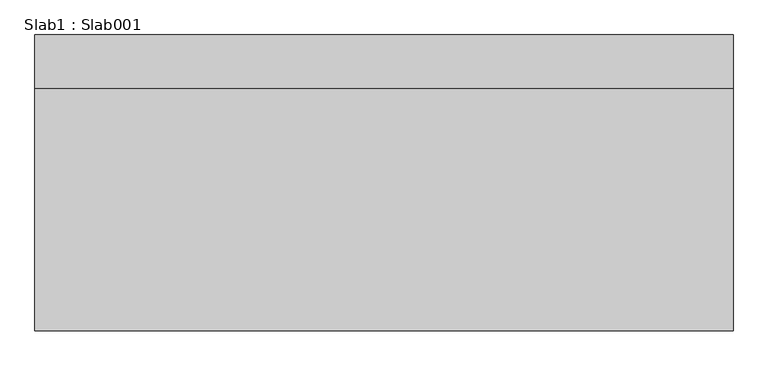
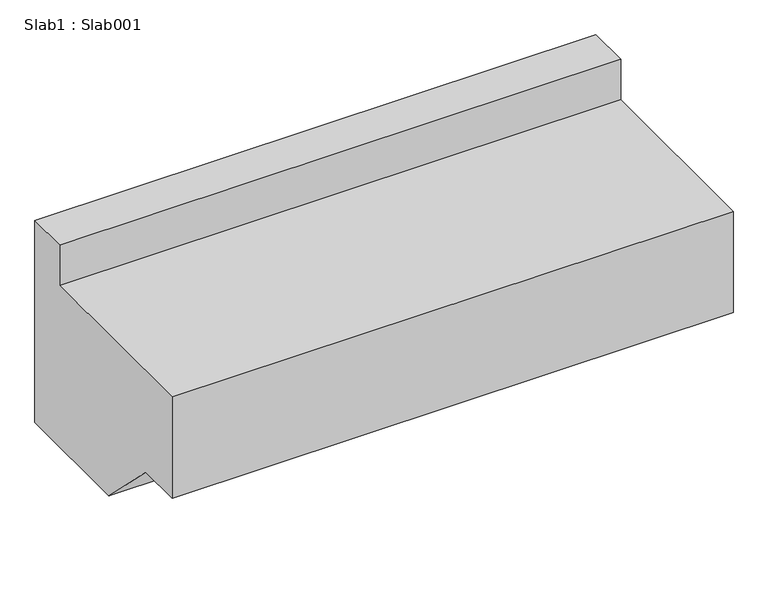
"""IFC4 building model written with IfcOpenShell, lengths in millimetres: proxy geometry, Slab1 : Slab001."""

from ifc_helpers import new_model, si_unit, frame, origin, place, context, project, spatial, polyline, outline, extrude, source, transform, mapped, element, save


def slab1_slab001_80c4c31f(model_context):
    return source(origin(), model_context, "Body", "SweptSolid", [
        extrude(outline(polyline([(9596.9851979, 36531.296), (9596.9851979, 36683.696), (9749.3851979, 36683.696), (9749.3851979, 35921.696), (9292.1851979, 35921.696), (9063.5851979, 36150.296), (8902.0438813, 36150.296), (8902.0438813, 36531.296), (9596.9851979, 36531.296)])), frame((3694.2883192, 0.0, 0.0), z_axis=(1.0, 0.0, 0.0), x_axis=(0.0, 1.0, 0.0)), (0.0, 0.0, 1.0), 2000.0),
    ])


if __name__ == "__main__":
    model = new_model("IFC4")
    model_context = context("Model", 3, world=origin())
    ifc_project = project(units=[si_unit("LENGTHUNIT", "METRE", prefix="MILLI")], contexts=[model_context])
    site = spatial("IfcSite", under=ifc_project)
    building = spatial("IfcBuilding", under=site)
    placement = place(None, origin())
    slab1_slab001_shape = slab1_slab001_80c4c31f(model_context)
    element("IfcBuildingElementProxy", 1, Name="Slab1 : Slab001", ObjectType="Slab1 : Slab001", at=placement, inside=building, context=model_context, shape_type="MappedRepresentation", body=[
        mapped(slab1_slab001_shape, transform((0.0, 0.0, 0.0), x_axis=(1.0, 0.0, 0.0), y_axis=(0.0, 1.0, 0.0), z_axis=(0.0, 0.0, 1.0))),
    ])
    save(model, "model.ifc")

# Revit data of these elements
# Type "Slab1 : Slab001"
#   NameOverride = "Slab001"
# Element 1 (IfcBuildingElementProxy, "Slab1 : Slab001")
#   Materials on its faces: "CONCRETE SLAB W/ GRADE BEAM (SEE STRUCT DWGS)"
# Materials
#   "CONCRETE SLAB W/ GRADE BEAM (SEE STRUCT DWGS)": class "Unassigned", colour RGB 128 128 128, transparency 0, Cost = 0
